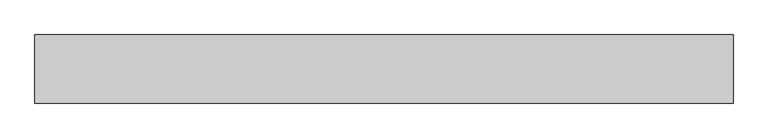
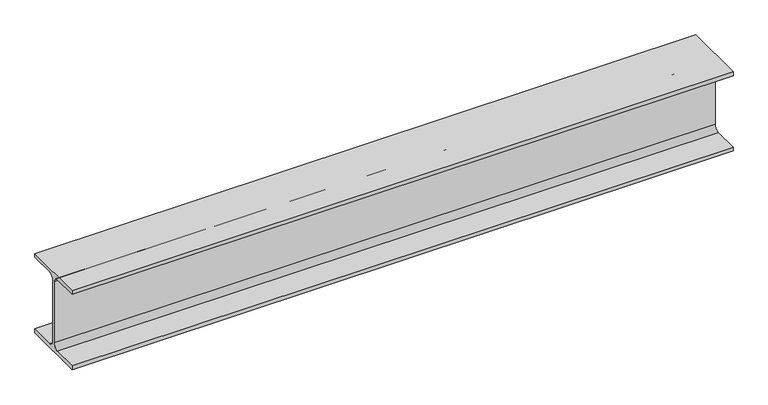
"""IFC4 building model written with IfcOpenShell, lengths in millimetres: beam geometry, 0912_Steel Framing_H-KSD3502 : H_SB_ASB_H-194x150x6x9."""

import ifcopenshell
import ifcopenshell.guid

model = None  # the IFC model being written
_history = None  # IfcOwnerHistory: only IFC2X3 demands one
_inside = {}  # id of a spatial element -> (the spatial element, [elements in it])
_under = {}  # id of a project, library or spatial element -> (it, [spatial elements below it])
_declared = {}  # id of a project -> (the project, [libraries it declares])
_typed = {}  # id of a type object -> (the type object, [elements of that type])
_made_of = {}  # id of a material, layer set ... -> (it, [elements and type objects made of it])


def new_model(schema):
    """Start an empty IFC model of exactly this schema.

    Asked for "IFC4X3", IfcOpenShell would pick the latest addendum, in which some entities
    have other attributes; the version numbers below select the first issue.
    IFC2X3 requires an IfcOwnerHistory on every rooted entity: one is made here for all.
    """
    global model, _history
    if schema == "IFC4X3":
        model = ifcopenshell.file(schema_version=(4, 3, 0, 0))
    else:
        model = ifcopenshell.file(schema=schema)
    _inside.clear()
    _under.clear()
    _declared.clear()
    _typed.clear()
    _made_of.clear()
    _history = None
    if model.schema == "IFC2X3":
        org = make("IfcOrganization", Name="unknown")
        user = make(
            "IfcPersonAndOrganization",
            ThePerson=make("IfcPerson", FamilyName="unknown"),
            TheOrganization=org,
        )
        app = make(
            "IfcApplication",
            ApplicationDeveloper=org,
            Version="unknown",
            ApplicationFullName="unknown",
            ApplicationIdentifier="unknown",
        )
        _history = make(
            "IfcOwnerHistory",
            OwningUser=user,
            OwningApplication=app,
            ChangeAction="ADDED",
            CreationDate=0,
        )
    return model


def make(cls, **values):
    """One entity of the class cls with the attributes given. An attribute that is None is left unset."""
    return model.create_entity(
        cls, **{name: value for name, value in values.items() if value is not None}
    )


def rooted(cls, **values):
    """An entity with a GlobalId (a new one), such as an element, a storey or a relation."""
    return make(cls, GlobalId=ifcopenshell.guid.new(), OwnerHistory=_history, **values)


def si_unit(unit_type, name, prefix=None):
    """IfcSIUnit, for example si_unit("LENGTHUNIT", "METRE", prefix="MILLI")."""
    return make("IfcSIUnit", UnitType=unit_type, Prefix=prefix, Name=name)


def assignment(units):
    """IfcUnitAssignment: the units of a project."""
    return None if units is None else make("IfcUnitAssignment", Units=units)


def point(xyz):
    """IfcCartesianPoint."""
    return None if xyz is None else make("IfcCartesianPoint", Coordinates=xyz)


def direction(xyz):
    """IfcDirection."""
    return None if xyz is None else make("IfcDirection", DirectionRatios=xyz)


def frame(location, z_axis=None, x_axis=None):
    """IfcAxis2Placement3D, a coordinate frame: its origin and axes. An axis left out is left unset."""
    return make(
        "IfcAxis2Placement3D",
        Location=point(location),
        Axis=direction(z_axis),
        RefDirection=direction(x_axis),
    )


def frame_2d(location, x_axis=None):
    """IfcAxis2Placement2D, a coordinate frame in the plane: its origin and x axis."""
    return make(
        "IfcAxis2Placement2D", Location=point(location), RefDirection=direction(x_axis)
    )


def origin():
    """The frame at (0, 0, 0) with its axes left unset."""
    return frame((0.0, 0.0, 0.0))


def place(relative_to, where):
    """IfcLocalPlacement: puts the frame where relative to a parent placement (None: the world)."""
    return make(
        "IfcLocalPlacement", PlacementRelTo=relative_to, RelativePlacement=where
    )


def context(
    kind, dimensions, precision=None, world=None, true_north=None, identifier=None
):
    """IfcGeometricRepresentationContext, for example the 3D "Model" context."""
    return make(
        "IfcGeometricRepresentationContext",
        ContextIdentifier=identifier,
        ContextType=kind,
        CoordinateSpaceDimension=dimensions,
        Precision=precision,
        WorldCoordinateSystem=world,
        TrueNorth=true_north,
    )


def project(units=None, contexts=None):
    """IfcProject with its units and contexts."""
    return rooted(
        "IfcProject",
        Name="project",
        RepresentationContexts=contexts,
        UnitsInContext=assignment(units),
    )


def spatial(cls, under=None, at=None, **own):
    """A site, building, storey or space (cls), placed at a placement, below another one or the project."""
    s = rooted(cls, ObjectPlacement=at, **own)
    if under is not None:
        _under.setdefault(under.id(), (under, []))[1].append(s)
    return s


def polyline(points):
    """IfcPolyline through the points."""
    return make("IfcPolyline", Points=[point(p) for p in points])


def circle_curve(where, radius):
    """IfcCircle in the frame where."""
    return make("IfcCircle", Position=where, Radius=radius)


def trimmed(basis, trim1, trim2, sense, master):
    """IfcTrimmedCurve: the piece of a basis curve between two trims."""
    return make(
        "IfcTrimmedCurve",
        BasisCurve=basis,
        Trim1=trim1,
        Trim2=trim2,
        SenseAgreement=sense,
        MasterRepresentation=master,
    )


def segment(curve, same_sense, transition):
    """IfcCompositeCurveSegment."""
    return make(
        "IfcCompositeCurveSegment",
        Transition=transition,
        SameSense=same_sense,
        ParentCurve=curve,
    )


def composite_curve(segments, self_intersect=None):
    """IfcCompositeCurve: segments joined end to end."""
    return make("IfcCompositeCurve", Segments=segments, SelfIntersect=self_intersect)


def outline(outer, holes=None, kind="AREA"):
    """IfcArbitraryClosedProfileDef: a profile drawn as a closed curve; with holes, ...WithVoids."""
    if holes is None:
        return make("IfcArbitraryClosedProfileDef", ProfileType=kind, OuterCurve=outer)
    return make(
        "IfcArbitraryProfileDefWithVoids",
        ProfileType=kind,
        OuterCurve=outer,
        InnerCurves=holes,
    )


def extrude(swept, where, along, depth):
    """IfcExtrudedAreaSolid: the profile swept, set in the frame where, extruded along a direction by depth."""
    return make(
        "IfcExtrudedAreaSolid",
        SweptArea=swept,
        Position=where,
        ExtrudedDirection=direction(along),
        Depth=depth,
    )


def shape(context_of_items, identifier, shape_type, items):
    """IfcShapeRepresentation: the items that make up one representation, for example the "Body"."""
    return make(
        "IfcShapeRepresentation",
        ContextOfItems=context_of_items,
        RepresentationIdentifier=identifier,
        RepresentationType=shape_type,
        Items=items,
    )


def source(mapping_origin, context_of_items, identifier, shape_type, items):
    """IfcRepresentationMap: a shape defined once, which mapped items show again and again."""
    return make(
        "IfcRepresentationMap",
        MappingOrigin=mapping_origin,
        MappedRepresentation=shape(context_of_items, identifier, shape_type, items),
    )


def transform(
    local_origin,
    x_axis=None,
    y_axis=None,
    z_axis=None,
    scale=None,
    scale2=None,
    scale3=None,
    uniform=True,
):
    """IfcCartesianTransformationOperator3D, or its non-uniform kind. x_axis, y_axis, z_axis: its Axis1, 2, 3."""
    if uniform:
        return make(
            "IfcCartesianTransformationOperator3D",
            Axis1=direction(x_axis),
            Axis2=direction(y_axis),
            LocalOrigin=point(local_origin),
            Scale=scale,
            Axis3=direction(z_axis),
        )
    return make(
        "IfcCartesianTransformationOperator3DnonUniform",
        Axis1=direction(x_axis),
        Axis2=direction(y_axis),
        LocalOrigin=point(local_origin),
        Scale=scale,
        Axis3=direction(z_axis),
        Scale2=scale2,
        Scale3=scale3,
    )


def mapped(mapping_source, mapping_target):
    """IfcMappedItem: shows the shape of a source again, moved by a transform."""
    return make(
        "IfcMappedItem", MappingSource=mapping_source, MappingTarget=mapping_target
    )


def made_of(thing, what):
    """Note that an element or type object is made of a material, layer set ...; save() writes the relation."""
    if what is not None:
        _made_of.setdefault(what.id(), (what, []))[1].append(thing)
    return thing


def element(
    cls,
    number,
    at=None,
    inside=None,
    cuts=None,
    type_object=None,
    material=None,
    context=None,
    identifier="Body",
    shape_type=None,
    held_by="IfcProductDefinitionShape",
    body=None,
    shapes=None,
    **own,
):
    """One element of the class cls, such as IfcWall. Its Tag is "e" and its number.

    at: its placement. inside: the storey or other place that contains it. cuts: it is an
    opening in that element (IfcRelVoidsElement). A single representation is given by context,
    identifier, shape_type and body (its items); several are given by shapes. held_by: the class
    of the entity that holds the representations. save() writes the other relations.
    """
    e = rooted(cls, Tag="e%d" % number, ObjectPlacement=at, **own)
    if body is not None:
        shapes = [shape(context, identifier, shape_type, body)]
    if shapes is not None:
        e.Representation = make(held_by, Representations=shapes)
    if inside is not None:
        _inside.setdefault(inside.id(), (inside, []))[1].append(e)
    if cuts is not None:
        rooted(
            "IfcRelVoidsElement", RelatingBuildingElement=cuts, RelatedOpeningElement=e
        )
    if type_object is not None:
        _typed.setdefault(type_object.id(), (type_object, []))[1].append(e)
    return made_of(e, material)


def aggregate(whole, parts):
    """IfcRelAggregates: a whole, such as a stair, and the parts it consists of."""
    return rooted("IfcRelAggregates", RelatingObject=whole, RelatedObjects=parts)


def save(model, path):
    """Write the relations noted so far, then the file.

    IfcRelAggregates (storeys below a building ...), IfcRelContainedInSpatialStructure (elements
    in a storey), IfcRelDefinesByType, IfcRelAssociatesMaterial and IfcRelDeclares: one each for
    every whole, place, type object, material and project.
    """
    for whole, parts in _under.values():
        aggregate(whole, parts)
    for where, things in _inside.values():
        rooted(
            "IfcRelContainedInSpatialStructure",
            RelatedElements=things,
            RelatingStructure=where,
        )
    for kind, things in _typed.values():
        rooted("IfcRelDefinesByType", RelatedObjects=things, RelatingType=kind)
    for what, things in _made_of.values():
        rooted("IfcRelAssociatesMaterial", RelatedObjects=things, RelatingMaterial=what)
    for by, libraries in _declared.values():
        rooted("IfcRelDeclares", RelatingContext=by, RelatedDefinitions=libraries)
    model.write(path)


def beam_7cd79bbf(model_context):
    return source(origin(), model_context, "Body", "SweptSolid", [
        extrude(outline(composite_curve([segment(polyline([(-75.0, -88.0), (-16.0, -88.0)]), True, "CONTINUOUS"), segment(trimmed(circle_curve(frame_2d((-16.0, -75.0)), 13.0), [point((-16.0, -88.0))], [point((-3.0, -75.0))], True, "CARTESIAN"), True, "CONTINUOUS"), segment(polyline([(-3.0, -75.0), (-3.0, 75.0)]), True, "CONTINUOUS"), segment(trimmed(circle_curve(frame_2d((-16.0, 75.0)), 13.0), [point((-3.0, 75.0))], [point((-16.0, 88.0))], True, "CARTESIAN"), True, "CONTINUOUS"), segment(polyline([(-16.0, 88.0), (-75.0, 88.0), (-75.0, 97.0), (75.0, 97.0), (75.0, 88.0), (16.0, 88.0)]), True, "CONTINUOUS"), segment(trimmed(circle_curve(frame_2d((16.0, 75.0)), 13.0), [point((16.0, 88.0))], [point((3.0, 75.0))], True, "CARTESIAN"), True, "CONTINUOUS"), segment(polyline([(3.0, 75.0), (3.0, -75.0)]), True, "CONTINUOUS"), segment(trimmed(circle_curve(frame_2d((16.0, -75.0)), 13.0), [point((3.0, -75.0))], [point((16.0, -88.0))], True, "CARTESIAN"), True, "CONTINUOUS"), segment(polyline([(16.0, -88.0), (75.0, -88.0), (75.0, -97.0), (-75.0, -97.0), (-75.0, -88.0)]), True, "CONTINUOUS")], self_intersect=False)), frame((-549.6452709, 0.0, 0.0), z_axis=(1.0, 0.0, 0.0), x_axis=(0.0, 1.0, 0.0)), (0.0, 0.0, 1.0), 1537.9998794),
    ])


if __name__ == "__main__":
    model = new_model("IFC4")
    model_context = context("Model", 3, world=origin())
    ifc_project = project(units=[si_unit("LENGTHUNIT", "METRE", prefix="MILLI")], contexts=[model_context])
    site = spatial("IfcSite", under=ifc_project)
    building = spatial("IfcBuilding", under=site)
    placement = place(None, origin())
    beam_shape = beam_7cd79bbf(model_context)
    element("IfcBeam", 1, ObjectType="0912_Steel Framing_H-KSD3502 : H_SB_ASB_H-194x150x6x9", at=placement, inside=building, context=model_context, shape_type="MappedRepresentation", body=[
        mapped(beam_shape, transform((0.0, 0.0, 0.0), x_axis=(1.0, 0.0, 0.0), y_axis=(0.0, 1.0, 0.0), z_axis=(0.0, 0.0, 1.0))),
    ])
    save(model, "model.ifc")

# Revit data of these elements
# Type "0912_Steel Framing_H-KSD3502 : H_SB_ASB_H-194x150x6x9"
#   H_WM Code_1 = "S01AA002-00001 | Main Steel Structure Fabrication Work | Shelter/Building | Medium Steel - Standard (90KG/M>Weight≥30KG/M) | Material: (   )"
#   H_WM Code_2 = "S03AA028-00001 | Main Steel Structure Erection Work | Shelter/Building | Medium Steel (90KG/M>Weight≥30KG/M) | Material: (   )"
#   H_WM Code_3 = "S01AA010-00001 | Main Steel Structure Fabrication Work | Shelter/Building | Steel Painting/Coating | for Non-Fireproofed Steel Surface, Surface Preparation, Primer, Second & Final Coat | Material: (   )"
#   H_Q'ty Cal Type Tag = "SB-Q2"
#   Width = 15.0 cm
#   Web Thickness = 0.6 cm
#   Web Fillet = 1.3 cm
#   Warping Constant = 43316.0 cm⁶
#   W = 0
#   Torsional Moment of Inertia = 8.622 cm⁴
#   Section Area = 39.01 cm²
#   Plastic Modulus weak axis = 104.0 cm³
#   Plastic Modulus strong axis = 309.0 cm³
#   Perimeter = 0.95 m²/m
#   Nominal Weight = 30.60 kgf/m
#   Moment of Inertia weak axis = 507.00 cm⁴
#   Moment of Inertia strong axis = 2690.00 cm⁴
#   Height = 19.4 cm
#   Flange Thickness = 0.9 cm
#   Elastic Modulus weak axis = 67.6 cm³
#   Elastic Modulus strong axis = 277.0 cm³
#   Centroid Vertical = 9.7 cm
#   Centroid Horizontal = 7.5 cm
#   Ix = 26900000
#   Length [instance default] = 1.5240 m
#   Zx = 309000
#   b = 0.1500 m
#   h = 0.1940 m
#   r = 0.0130 m
#   s = 0.0060 m
#   t = 0.0090 m
#   A = 0.003901 m²
#   Structural Material [instance default] = Steel, 45-345
#   Assembly Code = ""
# Element 1 (IfcBeam, "0912_Steel Framing_H-KSD3502 : H_SB_ASB_H-194x150x6x9")
#   Structural Material = none
# Materials
#   "Steel, 45-345": class "Metal", colour RGB 189 187 185, transparency 0, Description = "Steel 345 MPa", Cost = 0
